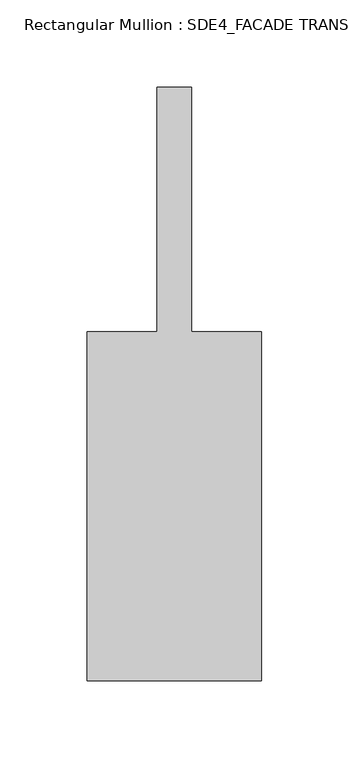
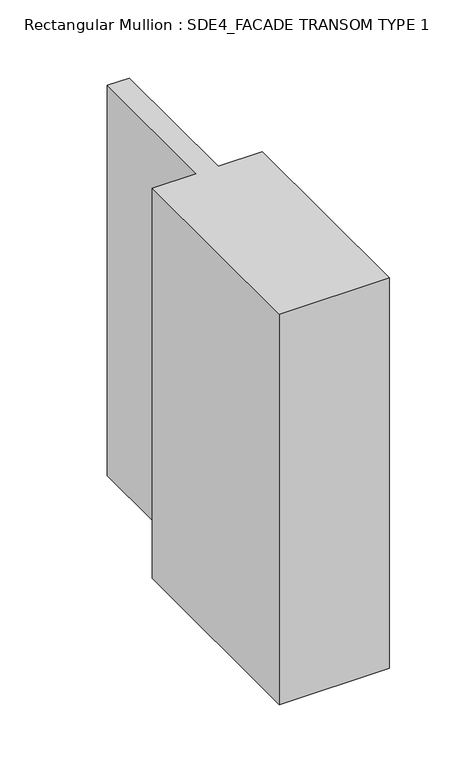
"""IFC4 building model written with IfcOpenShell, lengths in millimetres: member geometry, Rectangular Mullion : SDE4_FACADE TRANSOM TYPE 1."""

from ifc_helpers import new_model, si_unit, frame, origin, place, context, project, spatial, polyline, outline, extrude, source, transform, mapped, element, save


def rectangular_mullion_sde4_facade_transom_type_1_0ebbe2c6(model_context):
    return source(origin(), model_context, "Body", "SweptSolid", [
        extrude(outline(polyline([(50.0, -132.5), (-50.0, -132.5), (-50.0, 67.5), (-10.0, 67.5), (-10.0, 207.5), (10.0, 207.5), (10.0, 67.5), (50.0, 67.5), (50.0, -132.5)])), frame((0.0, 0.0, -375.304401), z_axis=(0.0, 0.0, 1.0), x_axis=(1.0, 0.0, 0.0)), (0.0, 0.0, 1.0), 375.304401),
    ])


if __name__ == "__main__":
    model = new_model("IFC4")
    model_context = context("Model", 3, world=origin())
    ifc_project = project(units=[si_unit("LENGTHUNIT", "METRE", prefix="MILLI")], contexts=[model_context])
    site = spatial("IfcSite", under=ifc_project)
    building = spatial("IfcBuilding", under=site)
    placement = place(None, origin())
    rectangular_mullion_sde4_facade_transom_type_1_shape = rectangular_mullion_sde4_facade_transom_type_1_0ebbe2c6(model_context)
    element("IfcMember", 1, ObjectType="Rectangular Mullion : SDE4_FACADE TRANSOM TYPE 1", at=placement, inside=building, context=model_context, shape_type="MappedRepresentation", body=[
        mapped(rectangular_mullion_sde4_facade_transom_type_1_shape, transform((0.0, 0.0, 0.0), x_axis=(1.0, 0.0, 0.0), y_axis=(0.0, 1.0, 0.0), z_axis=(0.0, 0.0, 1.0))),
    ])
    save(model, "model.ifc")

# Revit data of these elements
# Type "Rectangular Mullion : SDE4_FACADE TRANSOM TYPE 1"
#   built-in parameter 1007322 = 1.11549 (stored number, unit not read)
#   built-in parameter 1007321 = 0.164042 (stored number, unit not read)
#   built-in parameter 1007320 = 0.164042 (stored number, unit not read)
